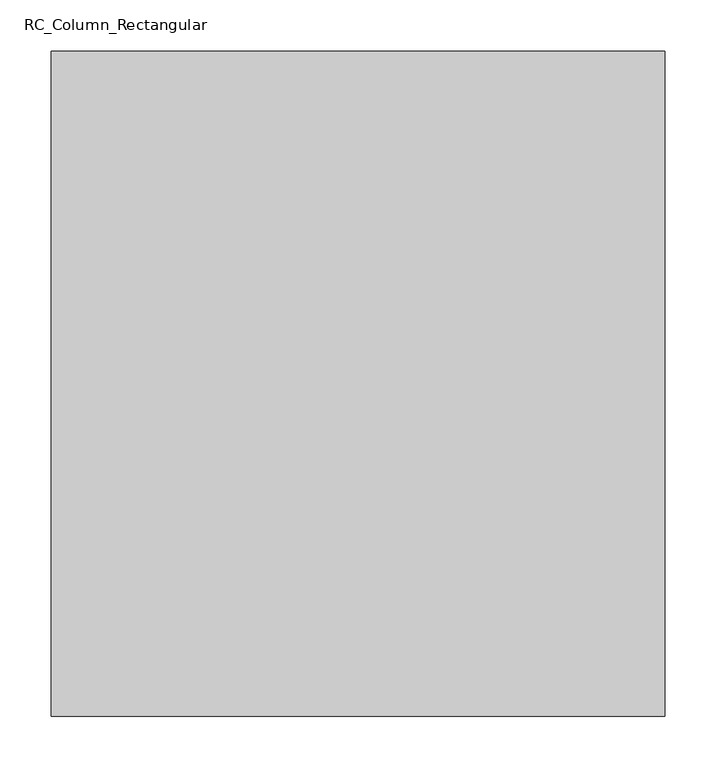
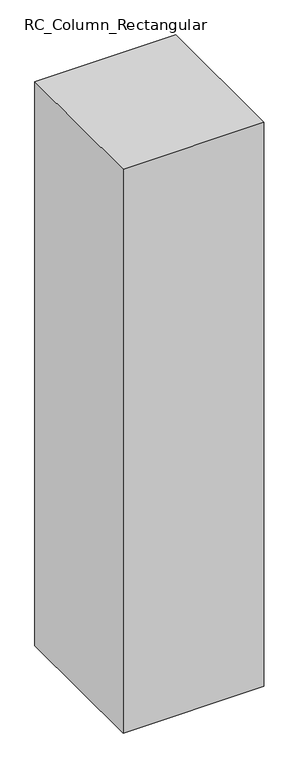
"""IFC4 building model written with IfcOpenShell, lengths in millimetres: column geometry, RC_Column_Rectangular : H_SC_AR_S15_AG Column_600x650_C3."""

from ifc_helpers import new_model, si_unit, frame, origin, place, context, project, spatial, polyline, outline, extrude, source, transform, mapped, element, save


def rc_column_rectangular_f1dd4ac0(model_context):
    return source(origin(), model_context, "Body", "SweptSolid", [
        extrude(outline(polyline([(300.0, 325.0), (300.0, -325.0), (-300.0, -325.0), (-300.0, 325.0), (300.0, 325.0)])), frame((0.0, 0.0, 4799.9618634), z_axis=(0.0, 0.0, 1.0), x_axis=(1.0, 0.0, 0.0)), (0.0, 0.0, 1.0), 2540.0381366),
    ])


if __name__ == "__main__":
    model = new_model("IFC4")
    model_context = context("Model", 3, world=origin())
    ifc_project = project(units=[si_unit("LENGTHUNIT", "METRE", prefix="MILLI")], contexts=[model_context])
    site = spatial("IfcSite", under=ifc_project)
    building = spatial("IfcBuilding", under=site)
    placement = place(None, origin())
    rc_column_rectangular_shape = rc_column_rectangular_f1dd4ac0(model_context)
    element("IfcColumn", 1, ObjectType="RC_Column_Rectangular : H_SC_AR_S15_AG Column_600x650_C3", at=placement, inside=building, context=model_context, shape_type="MappedRepresentation", body=[
        mapped(rc_column_rectangular_shape, transform((0.0, 0.0, 0.0), x_axis=(1.0, 0.0, 0.0), y_axis=(0.0, 1.0, 0.0), z_axis=(0.0, 0.0, 1.0))),
    ])
    save(model, "model.ifc")

# Revit data of these elements
# Type "RC_Column_Rectangular : H_SC_AR_S15_AG Column_600x650_C3"
#   Width = 600 mm
#   Length = 650 mm
#   hec_material3 [instance default] = none
#   hec_material2 [instance default] = none
#   hec_material1 [instance default] = none
#   Structural Material [instance default] = none
#   Description = (empty or 0)
# Element 1 (IfcColumn, "RC_Column_Rectangular : H_SC_AR_S15_AG Column_600x650_C3")
#   Structural Material = Concrete_f'c=28MPa(Cylender)
#   Materials on its faces: "Concrete_f'c=28MPa(Cylender)"
# Materials
#   "Concrete_f'c=28MPa(Cylender)": class "Concrete", colour RGB 176 176 176, transparency 0, Description = "Reinf. Conc.", Cost = 0, Image = Concrete.Cast-In-Place.Flat.Polished.Grey.jpg
